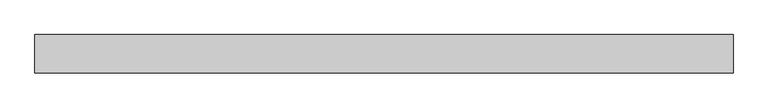
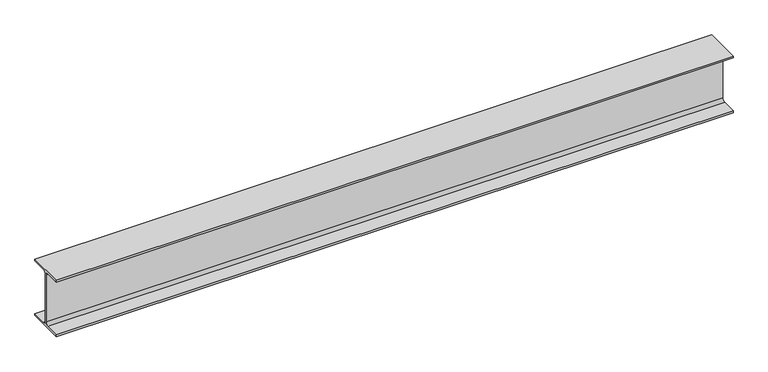
"""IFC4 building model written with IfcOpenShell, lengths in millimetres: beam geometry, 0912_Steel Framing_H-KSD3502 : H_SB_ASB_H-482x300x11x15."""

from ifc_helpers import new_model, si_unit, point, frame, frame_2d, origin, place, context, project, spatial, polyline, circle_curve, trimmed, segment, composite_curve, outline, extrude, source, transform, mapped, element, save


def beam_fac001ea(model_context):
    return source(origin(), model_context, "Body", "SweptSolid", [
        extrude(outline(composite_curve([segment(polyline([(150.0, -226.0), (150.0, -241.0), (-150.0, -241.0), (-150.0, -226.0), (-31.5, -226.0)]), True, "CONTINUOUS"), segment(trimmed(circle_curve(frame_2d((-31.5, -200.0)), 26.0), [point((-31.5, -226.0))], [point((-5.5, -200.0))], True, "CARTESIAN"), True, "CONTINUOUS"), segment(polyline([(-5.5, -200.0), (-5.5, 200.0)]), True, "CONTINUOUS"), segment(trimmed(circle_curve(frame_2d((-31.5, 200.0)), 26.0), [point((-5.5, 200.0))], [point((-31.5, 226.0))], True, "CARTESIAN"), True, "CONTINUOUS"), segment(polyline([(-31.5, 226.0), (-150.0, 226.0), (-150.0, 241.0), (150.0, 241.0), (150.0, 226.0), (31.5, 226.0)]), True, "CONTINUOUS"), segment(trimmed(circle_curve(frame_2d((31.5, 200.0)), 26.0), [point((31.5, 226.0))], [point((5.5, 200.0))], True, "CARTESIAN"), True, "CONTINUOUS"), segment(polyline([(5.5, 200.0), (5.5, -200.0)]), True, "CONTINUOUS"), segment(trimmed(circle_curve(frame_2d((31.5, -200.0)), 26.0), [point((5.5, -200.0))], [point((31.5, -226.0))], True, "CARTESIAN"), True, "CONTINUOUS"), segment(polyline([(31.5, -226.0), (150.0, -226.0)]), True, "CONTINUOUS")], self_intersect=False)), frame((-2837.3, 0.0, 0.0), z_axis=(1.0, 0.0, 0.0), x_axis=(0.0, 1.0, 0.0)), (0.0, 0.0, 1.0), 5474.6),
    ])


if __name__ == "__main__":
    model = new_model("IFC4")
    model_context = context("Model", 3, world=origin())
    ifc_project = project(units=[si_unit("LENGTHUNIT", "METRE", prefix="MILLI")], contexts=[model_context])
    site = spatial("IfcSite", under=ifc_project)
    building = spatial("IfcBuilding", under=site)
    placement = place(None, origin())
    beam_shape = beam_fac001ea(model_context)
    element("IfcBeam", 1, ObjectType="0912_Steel Framing_H-KSD3502 : H_SB_ASB_H-482x300x11x15", at=placement, inside=building, context=model_context, shape_type="MappedRepresentation", body=[
        mapped(beam_shape, transform((0.0, 0.0, 0.0), x_axis=(1.0, 0.0, 0.0), y_axis=(0.0, 1.0, 0.0), z_axis=(0.0, 0.0, 1.0))),
    ])
    save(model, "model.ifc")

# Revit data of these elements
# Type "0912_Steel Framing_H-KSD3502 : H_SB_ASB_H-482x300x11x15"
#   H_WM Code_1 = "S01AA001-00001 | Main Steel Structure Fabrication Work | Shelter/Building | Heavy Steel - Standard (Weight≥90KG/M) | Material: (   )"
#   H_WM Code_2 = "S03AA027-00001 | Main Steel Structure Erection Work | Shelter/Building | Heavy Steel (Weight≥90KG/M) | Material: (   )"
#   H_WM Code_3 = "S01AA010-00001 | Main Steel Structure Fabrication Work | Shelter/Building | Steel Painting/Coating | for Non-Fireproofed Steel Surface, Surface Preparation, Primer, Second & Final Coat | Material: (   )"
#   H_Q'ty Cal Type Tag = "SB-Q2"
#   Width = 30.0 cm
#   Web Thickness = 1.1 cm
#   Web Fillet = 2.6 cm
#   Warping Constant = 3680000.0 cm⁶
#   W = 0
#   Torsional Moment of Inertia = 88.2192 cm⁴
#   Section Area = 145.5 cm²
#   Plastic Modulus weak axis = 695.0 cm³
#   Plastic Modulus strong axis = 2790.0 cm³
#   Perimeter = 2.10 m²/m
#   Nominal Weight = 114.00 kgf/m
#   Moment of Inertia weak axis = 6760.00 cm⁴
#   Moment of Inertia strong axis = 60400.00 cm⁴
#   Height = 48.2 cm
#   Flange Thickness = 1.5 cm
#   Elastic Modulus weak axis = 451.0 cm³
#   Elastic Modulus strong axis = 2500.0 cm³
#   Centroid Vertical = 24.1 cm
#   Centroid Horizontal = 15.0 cm
#   Ix = 604000000
#   Length [instance default] = 1.5240 m
#   Zx = 2790000
#   b = 0.3000 m
#   h = 0.4820 m
#   r = 0.0260 m
#   s = 0.0110 m
#   t = 0.0150 m
#   A = 0.01455 m²
#   Structural Material [instance default] = Steel, 45-345
#   Assembly Code = ""
# Element 1 (IfcBeam, "0912_Steel Framing_H-KSD3502 : H_SB_ASB_H-482x300x11x15")
#   Structural Material = none
# Materials
#   "Steel, 45-345": class "Metal", colour RGB 189 187 185, transparency 0, Description = "Steel 345 MPa", Cost = 0
